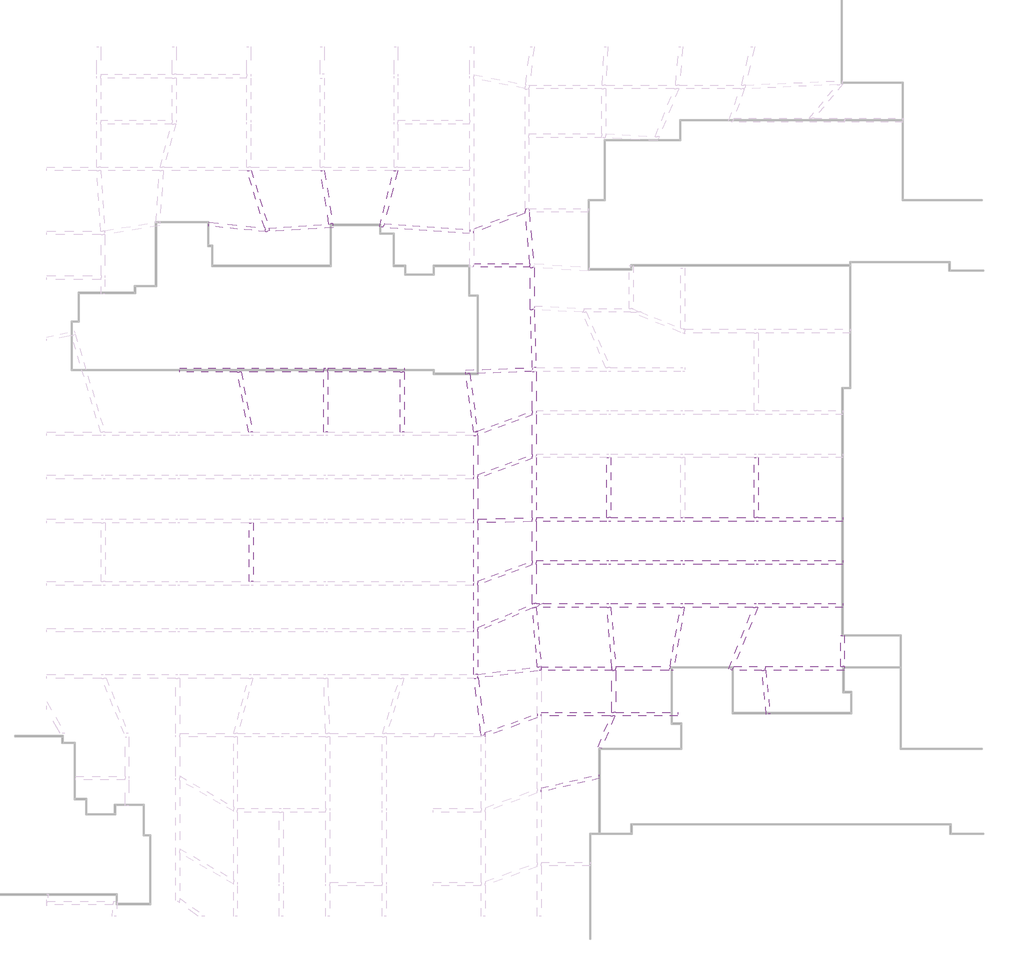
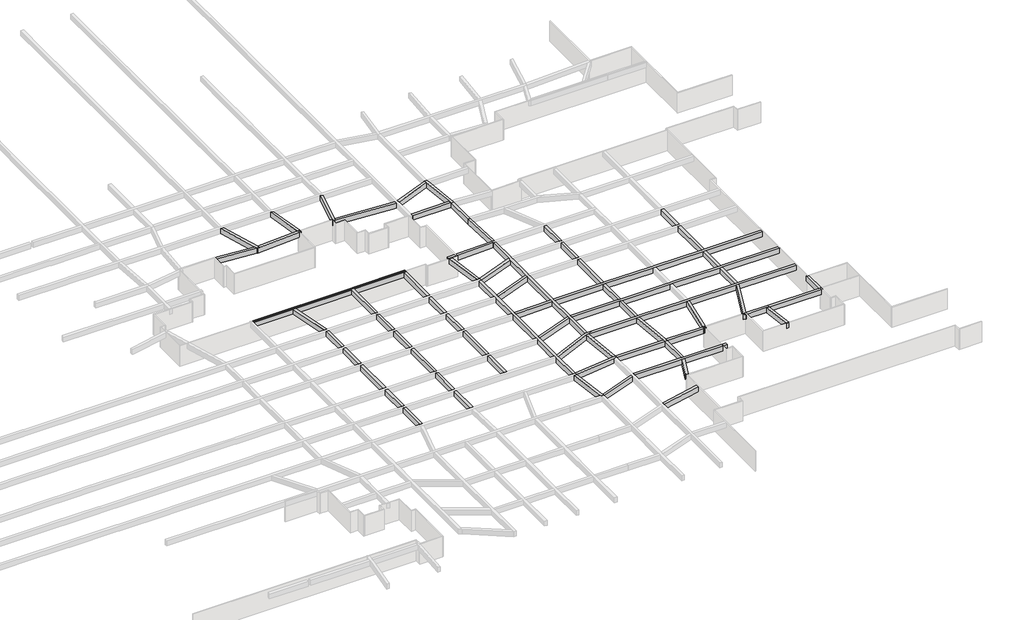
# One storey, part 23 of 45: 48 beams.
"""IFC4 building model written with IfcOpenShell, lengths in millimetres."""

from ifc_helpers import new_model, si_unit, frame, origin, place, context, project, spatial, polyline, outline, extrude, faceted_brep, element, save

model = new_model("IFC4")

# Units and contexts
model_context = context("Model", 3, world=origin())
ifc_project = project(units=[si_unit("LENGTHUNIT", "METRE", prefix="MILLI")], contexts=[model_context])

# Site, building, storey
site = spatial("IfcSite", under=ifc_project)
building = spatial("IfcBuilding", under=site)
storey = spatial("IfcBuildingStorey", under=building, Name="户型图", Elevation=0.0)

# Beams
placement = place(None, origin())
element("IfcBeam", 1, ObjectType="混凝土 - 矩形梁 : KL_beam", at=placement, inside=storey, context=model_context, shape_type="Brep", body=[
    faceted_brep([(31153.9230726, -39503.2652038, 3300.0), (30648.1791725, -33722.5859731, 3300.0), (30613.5574676, -33326.8580756, 3300.0), (30213.5574676, -33344.3224528, 3300.0), (30217.5432201, -33389.8798118, 3300.0), (30253.8104481, -33804.4161248, 3300.0), (30715.2619075, -39078.8304418, 3300.0), (30750.2573729, -39478.8304418, 3300.0), (30753.9230726, -39520.7295809, 3300.0), (30213.5574676, -33344.3224528, 2500.0), (30217.5432201, -33389.8798118, 2500.0), (30253.8104481, -33804.4161248, 2500.0), (30715.2619075, -39078.8304418, 2500.0), (30750.2573729, -39478.8304418, 2500.0), (30753.9230726, -39520.7295809, 2500.0), (30613.5574676, -33326.8580756, 2500.0), (30648.1791725, -33722.5859731, 2500.0), (31153.9230726, -39503.2652038, 2500.0)], [[[0, 1, 2, 3, 4, 5, 6, 7, 8]], [[8, 7, 6, 5, 4, 3, 9, 10, 11, 12, 13, 14]], [[14, 13, 12, 11, 10, 9, 15, 16, 17]], [[2, 1, 0, 17, 16, 15]], [[2, 15, 9, 3]], [[0, 8, 14, 17]]]),
])
element("IfcBeam", 2, ObjectType="混凝土 - 矩形梁 : KL_beam", at=placement, inside=storey, context=model_context, shape_type="Brep", body=[
    faceted_brep([(31153.9230726, -39503.2652038, 3300.0), (30753.9230726, -39520.7295809, 3300.0), (30753.9230726, -43901.7903057, 3300.0), (30760.4408066, -43902.1318857, 3300.0), (31153.9230726, -43922.7534174, 3300.0), (31153.9230726, -43522.204479, 3300.0), (30753.9230726, -39520.7295809, 2500.0), (30753.9230726, -43901.7903057, 2500.0), (31153.9230726, -39503.2652038, 2500.0), (31153.9230726, -43522.204479, 2500.0), (31153.9230726, -43922.7534174, 2500.0), (30760.4408066, -43902.1318857, 2500.0)], [[[0, 1, 2, 3, 4, 5]], [[1, 6, 7, 2]], [[6, 8, 9, 10, 11, 7]], [[8, 0, 5, 4, 10, 9]], [[0, 8, 6, 1]], [[4, 3, 2, 7, 11, 10]]]),
])
element("IfcBeam", 3, ObjectType="混凝土 - 矩形梁 : KL_beam", at=placement, inside=storey, context=model_context, shape_type="SweptSolid", body=[
    extrude(outline(polyline([(1338.0119922, -57112.697306), (1738.0119922, -57112.697306), (1738.0119922, -61244.2645659), (1338.0119922, -61244.2645659), (1338.0119922, -57112.697306)])), frame((0.0, 0.0, 2500.0), z_axis=(0.0, 0.0, 1.0), x_axis=(1.0, 0.0, 0.0)), (0.0, 0.0, 1.0), 800.0),
    extrude(outline(polyline([(1738.0119922, -82134.4617231), (1338.0119922, -82134.4617231), (1338.0119922, -77689.9052253), (1738.0119922, -77689.9052253), (1738.0119922, -82134.4617231)])), frame((0.0, 0.0, 2500.0), z_axis=(0.0, 0.0, 1.0), x_axis=(1.0, 0.0, 0.0)), (0.0, 0.0, 1.0), 800.0),
    extrude(outline(polyline([(1338.0119922, -61644.2645659), (1738.0119922, -61644.2645659), (1738.0119922, -65862.2662437), (1338.0119922, -65862.2662437), (1338.0119922, -61644.2645659)])), frame((0.0, 0.0, 2500.0), z_axis=(0.0, 0.0, 1.0), x_axis=(1.0, 0.0, 0.0)), (0.0, 0.0, 1.0), 800.0),
    extrude(outline(polyline([(1338.0119922, -66262.2662437), (1738.0119922, -66262.2662437), (1738.0119922, -72411.6769994), (1338.0119922, -72411.6769994), (1338.0119922, -66262.2662437)])), frame((0.0, 0.0, 2500.0), z_axis=(0.0, 0.0, 1.0), x_axis=(1.0, 0.0, 0.0)), (0.0, 0.0, 1.0), 800.0),
    extrude(outline(polyline([(1338.0119922, -72811.6769994), (1738.0119922, -72811.6769994), (1738.0119922, -77289.9052253), (1338.0119922, -77289.9052253), (1338.0119922, -72811.6769994)])), frame((0.0, 0.0, 2500.0), z_axis=(0.0, 0.0, 1.0), x_axis=(1.0, 0.0, 0.0)), (0.0, 0.0, 1.0), 800.0),
])
element("IfcBeam", 4, ObjectType="混凝土 - 矩形梁 : KL_beam", at=placement, inside=storey, context=model_context, shape_type="Brep", body=[
    faceted_brep([(9138.0119922, -82134.4617231, 3300.0), (9538.0119922, -82134.4617231, 3300.0), (9538.0119922, -77689.9052253, 3300.0), (9138.0119922, -77689.9052253, 3300.0), (9538.0119922, -82134.4617231, 2500.0), (9538.0119922, -77689.9052253, 2500.0), (9138.0119922, -82134.4617231, 2500.0), (9138.0119922, -77689.9052253, 2500.0)], [[[0, 1, 2, 3]], [[1, 4, 5, 2]], [[4, 6, 7, 5]], [[6, 0, 3, 7]], [[1, 0, 6, 4]], [[3, 2, 5, 7]]]),
    faceted_brep([(9138.0119922, -57112.697306, 3300.0), (9538.0119922, -57112.697306, 3300.0), (9538.0119922, -57112.697306, 2500.0), (9138.0119922, -57112.697306, 2500.0), (9538.0119922, -61244.2645659, 3300.0), (9138.0119922, -61244.2645659, 3300.0), (9138.0119922, -61244.2645659, 2500.0), (9538.0119922, -61244.2645659, 2500.0)], [[[0, 1, 2, 3]], [[4, 5, 6, 7]], [[1, 0, 5, 4]], [[2, 1, 4, 7]], [[3, 2, 7, 6]], [[0, 3, 6, 5]]]),
    faceted_brep([(9538.0119922, -56712.697306, 3300.0), (9138.0119922, -56712.697306, 3300.0), (9138.0119922, -56712.697306, 2500.0), (9538.0119922, -56712.697306, 2500.0), (9538.0119922, -50434.4617231, 3300.0), (9538.0119922, -50034.4617231, 3300.0), (9138.0119922, -50034.4617231, 3300.0), (9138.0119922, -50434.4617231, 3300.0), (9538.0119922, -50434.4617231, 2500.0), (9538.0119922, -50034.4617231, 2500.0), (9138.0119922, -50434.4617231, 2500.0), (9138.0119922, -50034.4617231, 2500.0)], [[[0, 1, 2, 3]], [[1, 0, 4, 5, 6, 7]], [[0, 3, 8, 9, 5, 4]], [[3, 2, 10, 11, 9, 8]], [[2, 1, 7, 6, 11, 10]], [[6, 5, 9, 11]]]),
    faceted_brep([(9138.0119922, -61644.2645659, 3300.0), (9538.0119922, -61644.2645659, 3300.0), (9538.0119922, -61644.2645659, 2500.0), (9138.0119922, -61644.2645659, 2500.0), (9538.0119922, -65862.2662437, 3300.0), (9138.0119922, -65862.2662437, 3300.0), (9138.0119922, -65862.2662437, 2500.0), (9538.0119922, -65862.2662437, 2500.0)], [[[0, 1, 2, 3]], [[4, 5, 6, 7]], [[1, 0, 5, 4]], [[2, 1, 4, 7]], [[3, 2, 7, 6]], [[0, 3, 6, 5]]]),
    faceted_brep([(9138.0119922, -66262.2662437, 3300.0), (9538.0119922, -66262.2662437, 3300.0), (9538.0119922, -66262.2662437, 2500.0), (9138.0119922, -66262.2662437, 2500.0), (9538.0119922, -72411.6769994, 3300.0), (9138.0119922, -72411.6769994, 3300.0), (9138.0119922, -72411.6769994, 2500.0), (9538.0119922, -72411.6769994, 2500.0)], [[[0, 1, 2, 3]], [[4, 5, 6, 7]], [[1, 0, 5, 4]], [[2, 1, 4, 7]], [[3, 2, 7, 6]], [[0, 3, 6, 5]]]),
    faceted_brep([(9138.0119922, -72811.6769994, 3300.0), (9538.0119922, -72811.6769994, 3300.0), (9538.0119922, -72811.6769994, 2500.0), (9138.0119922, -72811.6769994, 2500.0), (9538.0119922, -77289.9052253, 3300.0), (9138.0119922, -77289.9052253, 3300.0), (9138.0119922, -77289.9052253, 2500.0), (9538.0119922, -77289.9052253, 2500.0)], [[[0, 1, 2, 3]], [[4, 5, 6, 7]], [[1, 0, 5, 4]], [[2, 1, 4, 7]], [[3, 2, 7, 6]], [[0, 3, 6, 5]]]),
])
element("IfcBeam", 5, ObjectType="混凝土 - 矩形梁 : KL_beam", at=placement, inside=storey, context=model_context, shape_type="Brep", body=[
    faceted_brep([(17560.5867178, -50434.4617231, 3300.0), (17560.5867178, -50034.4617231, 3300.0), (9538.0119922, -50034.4617231, 3300.0), (9538.0119922, -50434.4617231, 3300.0), (17160.5867178, -50434.4617231, 3300.0), (17560.5867178, -50434.4617231, 2500.0), (9538.0119922, -50434.4617231, 2500.0), (17160.5867178, -50434.4617231, 2500.0), (17560.5867178, -50034.4617231, 2500.0), (9538.0119922, -50034.4617231, 2500.0)], [[[0, 1, 2, 3, 4]], [[5, 0, 4, 3, 6, 7]], [[8, 5, 7, 6, 9]], [[1, 8, 9, 2]], [[3, 2, 9, 6]], [[1, 0, 5, 8]]]),
])
element("IfcBeam", 6, ObjectType="混凝土 - 矩形梁 : KL_beam", at=placement, inside=storey, context=model_context, shape_type="Brep", body=[
    faceted_brep([(-5961.9880078, -50034.4617231, 3300.0), (-5961.9880078, -50434.4617231, 3300.0), (74.9529241, -50434.4617231, 3300.0), (482.4396021, -50434.4617231, 3300.0), (9138.0119922, -50434.4617231, 3300.0), (9138.0119922, -50034.4617231, 3300.0), (-5961.9880078, -50034.4617231, 2500.0), (9138.0119922, -50034.4617231, 2500.0), (-5961.9880078, -50434.4617231, 2500.0), (9138.0119922, -50434.4617231, 2500.0), (482.4396021, -50434.4617231, 2500.0), (74.9529241, -50434.4617231, 2500.0)], [[[0, 1, 2, 3, 4, 5]], [[6, 0, 5, 7]], [[8, 6, 7, 9, 10, 11]], [[1, 8, 11, 10, 9, 4, 3, 2]], [[1, 0, 6, 8]], [[5, 4, 9, 7]]]),
])
element("IfcBeam", 7, ObjectType="混凝土 - 矩形梁 : KL_beam", at=placement, inside=storey, context=model_context, shape_type="SweptSolid", body=[
    extrude(outline(polyline([(1702.8049756, -56712.697306), (1295.3182976, -56712.697306), (74.9529241, -50434.4617231), (482.4396021, -50434.4617231), (1702.8049756, -56712.697306)])), frame((0.0, 0.0, 2500.0), z_axis=(0.0, 0.0, 1.0), x_axis=(1.0, 0.0, 0.0)), (0.0, 0.0, 1.0), 800.0),
])
element("IfcBeam", 8, ObjectType="混凝土 - 矩形梁 : KL_beam", at=placement, inside=storey, context=model_context, shape_type="SweptSolid", body=[
    extrude(outline(polyline([(17560.5867178, -77289.9052253), (17160.5867178, -77289.9052253), (17160.5867178, -72811.6769994), (17560.5867178, -72811.6769994), (17560.5867178, -77289.9052253)])), frame((0.0, 0.0, 2500.0), z_axis=(0.0, 0.0, 1.0), x_axis=(1.0, 0.0, 0.0)), (0.0, 0.0, 1.0), 800.0),
    extrude(outline(polyline([(17160.5867178, -50434.4617231), (17560.5867178, -50434.4617231), (17560.5867178, -56712.697306), (17160.5867178, -56712.697306), (17160.5867178, -50434.4617231)])), frame((0.0, 0.0, 2500.0), z_axis=(0.0, 0.0, 1.0), x_axis=(1.0, 0.0, 0.0)), (0.0, 0.0, 1.0), 800.0),
    extrude(outline(polyline([(17160.5867178, -57112.697306), (17560.5867178, -57112.697306), (17560.5867178, -61244.2645659), (17160.5867178, -61244.2645659), (17160.5867178, -57112.697306)])), frame((0.0, 0.0, 2500.0), z_axis=(0.0, 0.0, 1.0), x_axis=(1.0, 0.0, 0.0)), (0.0, 0.0, 1.0), 800.0),
    extrude(outline(polyline([(17160.5867178, -61644.2645659), (17560.5867178, -61644.2645659), (17560.5867178, -65862.2662437), (17160.5867178, -65862.2662437), (17160.5867178, -61644.2645659)])), frame((0.0, 0.0, 2500.0), z_axis=(0.0, 0.0, 1.0), x_axis=(1.0, 0.0, 0.0)), (0.0, 0.0, 1.0), 800.0),
    extrude(outline(polyline([(17160.5867178, -66262.2662437), (17560.5867178, -66262.2662437), (17560.5867178, -72411.6769994), (17160.5867178, -72411.6769994), (17160.5867178, -66262.2662437)])), frame((0.0, 0.0, 2500.0), z_axis=(0.0, 0.0, 1.0), x_axis=(1.0, 0.0, 0.0)), (0.0, 0.0, 1.0), 800.0),
])
element("IfcBeam", 9, ObjectType="混凝土 - 矩形梁 : KL_beam", at=placement, inside=storey, context=model_context, shape_type="Brep", body=[
    faceted_brep([(25266.4388689, -57112.697306, 3300.0), (24866.4388689, -57112.697306, 3300.0), (24866.4388689, -61244.2645659, 3300.0), (24866.4388689, -61644.2645659, 3300.0), (24866.4388689, -65862.2662437, 3300.0), (24866.4388689, -66262.2662437, 3300.0), (24866.4388689, -72411.6769994, 3300.0), (24866.4388689, -72811.6769994, 3300.0), (24866.4388689, -77289.9052253, 3300.0), (24866.4388689, -77689.9052253, 3300.0), (24866.4388689, -82134.4617231, 3300.0), (25266.4388689, -82134.4617231, 3300.0), (25266.4388689, -82108.4028459, 3300.0), (25266.4388689, -77622.2823376, 3300.0), (25266.4388689, -77187.7381866, 3300.0), (25266.4388689, -72751.6932425, 3300.0), (25266.4388689, -72326.0221335, 3300.0), (25266.4388689, -66257.3977389, 3300.0), (25266.4388689, -65857.2762703, 3300.0), (25266.4388689, -61584.3060735, 3300.0), (25266.4388689, -61158.6349646, 3300.0), (25266.4388689, -57112.697306, 2500.0), (25266.4388689, -82134.4617231, 2500.0), (25266.4388689, -82108.4028459, 2500.0), (25266.4388689, -77622.2823376, 2500.0), (25266.4388689, -77187.7381866, 2500.0), (25266.4388689, -72751.6932425, 2500.0), (25266.4388689, -72326.0221335, 2500.0), (25266.4388689, -66257.3977389, 2500.0), (25266.4388689, -65857.2762703, 2500.0), (25266.4388689, -61584.3060735, 2500.0), (25266.4388689, -61158.6349646, 2500.0), (24866.4388689, -57112.697306, 2500.0), (24866.4388689, -82134.4617231, 2500.0), (24866.4388689, -77689.9052253, 2500.0), (24866.4388689, -77289.9052253, 2500.0), (24866.4388689, -72811.6769994, 2500.0), (24866.4388689, -72411.6769994, 2500.0), (24866.4388689, -66262.2662437, 2500.0), (24866.4388689, -65862.2662437, 2500.0), (24866.4388689, -61644.2645659, 2500.0), (24866.4388689, -61244.2645659, 2500.0)], [[[0, 1, 2, 3, 4, 5, 6, 7, 8, 9, 10, 11, 12, 13, 14, 15, 16, 17, 18, 19, 20]], [[21, 0, 20, 19, 18, 17, 16, 15, 14, 13, 12, 11, 22, 23, 24, 25, 26, 27, 28, 29, 30, 31]], [[32, 21, 31, 30, 29, 28, 27, 26, 25, 24, 23, 22, 33, 34, 35, 36, 37, 38, 39, 40, 41]], [[1, 32, 41, 40, 39, 38, 37, 36, 35, 34, 33, 10, 9, 8, 7, 6, 5, 4, 3, 2]], [[1, 0, 21, 32]], [[11, 10, 33, 22]]]),
])
element("IfcBeam", 10, ObjectType="混凝土 - 矩形梁 : KL_beam", at=placement, inside=storey, context=model_context, shape_type="Brep", body=[
    faceted_brep([(25031.1734727, -56712.697306, 3300.0), (25266.4388689, -56712.697306, 3300.0), (25266.4388689, -57052.7388136, 3300.0), (30980.1331881, -54973.1241538, 3300.0), (30980.1331881, -54547.4530448, 3300.0), (25230.8624807, -56640.016451, 3300.0), (25266.4388689, -57052.7388136, 2500.0), (30980.1331881, -54973.1241538, 2500.0), (25266.4388689, -56712.697306, 2500.0), (25031.1734727, -56712.697306, 2500.0), (25230.8624807, -56640.016451, 2500.0), (30980.1331881, -54547.4530448, 2500.0)], [[[0, 1, 2, 3, 4, 5]], [[2, 6, 7, 3]], [[8, 9, 10, 11, 7, 6]], [[9, 0, 5, 4, 11, 10]], [[8, 1, 0, 9]], [[1, 8, 6, 2]], [[4, 3, 7, 11]]]),
])
element("IfcBeam", 11, ObjectType="混凝土 - 矩形梁 : KL_beam", at=placement, inside=storey, context=model_context, shape_type="SweptSolid", body=[
    extrude(outline(polyline([(25266.4388689, -61584.3060735), (25266.4388689, -61158.6349646), (30980.1331881, -59079.0203047), (30980.1331881, -59504.6914136), (25266.4388689, -61584.3060735)])), frame((0.0, 0.0, 2500.0), z_axis=(0.0, 0.0, 1.0), x_axis=(1.0, 0.0, 0.0)), (0.0, 0.0, 1.0), 800.0),
])
element("IfcBeam", 12, ObjectType="混凝土 - 矩形梁 : KL_beam", at=placement, inside=storey, context=model_context, shape_type="SweptSolid", body=[
    extrude(outline(polyline([(25266.4388689, -66257.3977389), (25266.4388689, -65857.2762703), (30980.1331881, -65716.4554426), (30980.1331881, -66116.5769112), (25266.4388689, -66257.3977389)])), frame((0.0, 0.0, 2500.0), z_axis=(0.0, 0.0, 1.0), x_axis=(1.0, 0.0, 0.0)), (0.0, 0.0, 1.0), 800.0),
])
element("IfcBeam", 13, ObjectType="混凝土 - 矩形梁 : KL_beam", at=placement, inside=storey, context=model_context, shape_type="SweptSolid", body=[
    extrude(outline(polyline([(25266.4388689, -72751.6932425), (25266.4388689, -72326.0221335), (30980.1331881, -70246.4074737), (30980.1331881, -70672.0785826), (25266.4388689, -72751.6932425)])), frame((0.0, 0.0, 2500.0), z_axis=(0.0, 0.0, 1.0), x_axis=(1.0, 0.0, 0.0)), (0.0, 0.0, 1.0), 800.0),
])
element("IfcBeam", 14, ObjectType="混凝土 - 矩形梁 : KL_beam", at=placement, inside=storey, context=model_context, shape_type="Brep", body=[
    faceted_brep([(32124.8023079, -74711.0797773, 3300.0), (31380.1331881, -74711.0797773, 3300.0), (31101.0804418, -74711.0797773, 3300.0), (30980.1331881, -74762.4188406, 3300.0), (25266.4388689, -77187.7381866, 3300.0), (25266.4388689, -77622.2823376, 3300.0), (31001.9328556, -75187.7095817, 3300.0), (31182.4613615, -75111.0797773, 3300.0), (32124.8023079, -74711.0797773, 2500.0), (25266.4388689, -77622.2823376, 2500.0), (31001.9328556, -75187.7095817, 2500.0), (31182.4613615, -75111.0797773, 2500.0), (31101.0804418, -74711.0797773, 2500.0), (31380.1331881, -74711.0797773, 2500.0), (25266.4388689, -77187.7381866, 2500.0), (30980.1331881, -74762.4188406, 2500.0)], [[[0, 1, 2, 3, 4, 5, 6, 7]], [[8, 0, 7, 6, 5, 9, 10, 11]], [[12, 13, 8, 11, 10, 9, 14, 15]], [[2, 12, 15, 14, 4, 3]], [[5, 4, 14, 9]], [[2, 1, 0, 8, 13, 12]]]),
])
element("IfcBeam", 15, ObjectType="混凝土 - 矩形梁 : KL_beam", at=placement, inside=storey, context=model_context, shape_type="Brep", body=[
    faceted_brep([(25266.4388689, -82108.4028459, 3300.0), (25266.4388689, -82134.4617231, 3300.0), (25266.4388689, -82511.406776, 3300.0), (25289.3682002, -82508.5914082, 3300.0), (31516.4740744, -81743.9989477, 3300.0), (31916.4740744, -81694.8851233, 3300.0), (31931.3727413, -81693.0557971, 3300.0), (31916.4740744, -81509.5363909, 3300.0), (31900.9194594, -81317.9371223, 3300.0), (31898.9785552, -81294.0293728, 3300.0), (31501.6234284, -81342.8184476, 3300.0), (25266.4388689, -82511.406776, 2500.0), (25289.3682002, -82508.5914082, 2500.0), (31516.4740744, -81743.9989477, 2500.0), (31916.4740744, -81694.8851233, 2500.0), (31931.3727413, -81693.0557971, 2500.0), (25266.4388689, -82134.4617231, 2500.0), (25266.4388689, -82108.4028459, 2500.0), (31501.6234284, -81342.8184476, 2500.0), (31898.9785552, -81294.0293728, 2500.0), (31900.9194594, -81317.9371223, 2500.0), (31916.4740744, -81509.5363909, 2500.0)], [[[0, 1, 2, 3, 4, 5, 6, 7, 8, 9, 10]], [[2, 11, 12, 13, 14, 15, 6, 5, 4, 3]], [[11, 16, 17, 18, 19, 20, 21, 15, 14, 13, 12]], [[9, 19, 18, 17, 0, 10]], [[0, 17, 16, 11, 2, 1]], [[9, 8, 7, 6, 15, 21, 20, 19]]]),
])
element("IfcBeam", 16, ObjectType="混凝土 - 矩形梁 : KL_beam", at=placement, inside=storey, context=model_context, shape_type="Brep", body=[
    faceted_brep([(63459.1246226, -74711.0797773, 3300.0), (63459.1246226, -75111.0797773, 3300.0), (63459.1246226, -75111.0797773, 2500.0), (63459.1246226, -74711.0797773, 2500.0), (54624.1889168, -74711.0797773, 3300.0), (54224.1889168, -74711.0797773, 3300.0), (46924.1889168, -74711.0797773, 3300.0), (46524.1889168, -74711.0797773, 3300.0), (39180.1331881, -74711.0797773, 3300.0), (38780.1331881, -74711.0797773, 3300.0), (32124.8023079, -74711.0797773, 3300.0), (31182.4613615, -75111.0797773, 3300.0), (31397.0277867, -75111.0797773, 3300.0), (38795.7118136, -75111.0797773, 3300.0), (39197.0277867, -75111.0797773, 3300.0), (46485.8381983, -75111.0797773, 3300.0), (46892.008843, -75111.0797773, 3300.0), (54127.6767231, -75111.0797773, 3300.0), (54559.0906202, -75111.0797773, 3300.0), (31182.4613615, -75111.0797773, 2500.0), (31397.0277867, -75111.0797773, 2500.0), (38795.7118136, -75111.0797773, 2500.0), (39197.0277867, -75111.0797773, 2500.0), (46485.8381983, -75111.0797773, 2500.0), (46892.008843, -75111.0797773, 2500.0), (54127.6767231, -75111.0797773, 2500.0), (54559.0906202, -75111.0797773, 2500.0), (32124.8023079, -74711.0797773, 2500.0), (38780.1331881, -74711.0797773, 2500.0), (39180.1331881, -74711.0797773, 2500.0), (46524.1889168, -74711.0797773, 2500.0), (46924.1889168, -74711.0797773, 2500.0), (54224.1889168, -74711.0797773, 2500.0), (54624.1889168, -74711.0797773, 2500.0)], [[[0, 1, 2, 3]], [[1, 0, 4, 5, 6, 7, 8, 9, 10, 11, 12, 13, 14, 15, 16, 17, 18]], [[2, 1, 18, 17, 16, 15, 14, 13, 12, 11, 19, 20, 21, 22, 23, 24, 25, 26]], [[3, 2, 26, 25, 24, 23, 22, 21, 20, 19, 27, 28, 29, 30, 31, 32, 33]], [[0, 3, 33, 32, 31, 30, 29, 28, 27, 10, 9, 8, 7, 6, 5, 4]], [[11, 10, 27, 19]]]),
])
element("IfcBeam", 17, ObjectType="混凝土 - 矩形梁 : KL_beam", at=placement, inside=storey, context=model_context, shape_type="Brep", body=[
    faceted_brep([(63459.3057658, -70188.5460678, 3300.0), (63459.3057658, -70588.5460678, 3300.0), (63459.3057658, -70588.5460678, 2500.0), (63459.3057658, -70188.5460678, 2500.0), (54624.1889168, -70188.5460678, 3300.0), (54224.1889168, -70188.5460678, 3300.0), (46924.1889168, -70188.5460678, 3300.0), (46524.1889168, -70188.5460678, 3300.0), (39180.1331881, -70188.5460678, 3300.0), (38780.1331881, -70188.5460678, 3300.0), (31380.1331881, -70188.5460678, 3300.0), (31380.1331881, -70588.5460678, 3300.0), (38780.1331881, -70588.5460678, 3300.0), (39180.1331881, -70588.5460678, 3300.0), (46524.1889168, -70588.5460678, 3300.0), (46924.1889168, -70588.5460678, 3300.0), (54224.1889168, -70588.5460678, 3300.0), (54624.1889168, -70588.5460678, 3300.0), (31380.1331881, -70588.5460678, 2500.0), (38780.1331881, -70588.5460678, 2500.0), (39180.1331881, -70588.5460678, 2500.0), (46524.1889168, -70588.5460678, 2500.0), (46924.1889168, -70588.5460678, 2500.0), (54224.1889168, -70588.5460678, 2500.0), (54624.1889168, -70588.5460678, 2500.0), (31380.1331881, -70188.5460678, 2500.0), (38780.1331881, -70188.5460678, 2500.0), (39180.1331881, -70188.5460678, 2500.0), (46524.1889168, -70188.5460678, 2500.0), (46924.1889168, -70188.5460678, 2500.0), (54224.1889168, -70188.5460678, 2500.0), (54624.1889168, -70188.5460678, 2500.0)], [[[0, 1, 2, 3]], [[1, 0, 4, 5, 6, 7, 8, 9, 10, 11, 12, 13, 14, 15, 16, 17]], [[2, 1, 17, 16, 15, 14, 13, 12, 11, 18, 19, 20, 21, 22, 23, 24]], [[3, 2, 24, 23, 22, 21, 20, 19, 18, 25, 26, 27, 28, 29, 30, 31]], [[0, 3, 31, 30, 29, 28, 27, 26, 25, 10, 9, 8, 7, 6, 5, 4]], [[10, 25, 18, 11]]]),
])
element("IfcBeam", 18, ObjectType="混凝土 - 矩形梁 : KL_beam", at=placement, inside=storey, context=model_context, shape_type="Brep", body=[
    faceted_brep([(63459.3057658, -65711.9700913, 3300.0), (63459.3057658, -66111.9700913, 3300.0), (63459.3057658, -66111.9700913, 2500.0), (63459.3057658, -65711.9700913, 2500.0), (54624.1889168, -65711.9700913, 3300.0), (54224.1889168, -65711.9700913, 3300.0), (46924.1889168, -65711.9700913, 3300.0), (46524.1889168, -65711.9700913, 3300.0), (39180.1331881, -65711.9700913, 3300.0), (38780.1331881, -65711.9700913, 3300.0), (31380.1331881, -65711.9700913, 3300.0), (31380.1331881, -66111.9700913, 3300.0), (38780.1331881, -66111.9700913, 3300.0), (39180.1331881, -66111.9700913, 3300.0), (46524.1889168, -66111.9700913, 3300.0), (46924.1889168, -66111.9700913, 3300.0), (54224.1889168, -66111.9700913, 3300.0), (54624.1889168, -66111.9700913, 3300.0), (31380.1331881, -66111.9700913, 2500.0), (38780.1331881, -66111.9700913, 2500.0), (39180.1331881, -66111.9700913, 2500.0), (46524.1889168, -66111.9700913, 2500.0), (46924.1889168, -66111.9700913, 2500.0), (54224.1889168, -66111.9700913, 2500.0), (54624.1889168, -66111.9700913, 2500.0), (31380.1331881, -65711.9700913, 2500.0), (38780.1331881, -65711.9700913, 2500.0), (39180.1331881, -65711.9700913, 2500.0), (46524.1889168, -65711.9700913, 2500.0), (46924.1889168, -65711.9700913, 2500.0), (54224.1889168, -65711.9700913, 2500.0), (54624.1889168, -65711.9700913, 2500.0)], [[[0, 1, 2, 3]], [[1, 0, 4, 5, 6, 7, 8, 9, 10, 11, 12, 13, 14, 15, 16, 17]], [[2, 1, 17, 16, 15, 14, 13, 12, 11, 18, 19, 20, 21, 22, 23, 24]], [[3, 2, 24, 23, 22, 21, 20, 19, 18, 25, 26, 27, 28, 29, 30, 31]], [[0, 3, 31, 30, 29, 28, 27, 26, 25, 10, 9, 8, 7, 6, 5, 4]], [[10, 25, 18, 11]]]),
])
element("IfcBeam", 19, ObjectType="混凝土 - 矩形梁 : KL_beam", at=placement, inside=storey, context=model_context, shape_type="Brep", body=[
    faceted_brep([(31161.4184615, -43923.1462341, 3300.0), (31153.9230726, -43922.7534174, 3300.0), (30760.4408066, -43902.1318857, 3300.0), (30973.0187032, -49989.5663744, 3300.0), (31373.2625209, -49989.5663744, 3300.0), (30760.4408066, -43902.1318857, 2500.0), (30973.0187032, -49989.5663744, 2500.0), (31153.9230726, -43922.7534174, 2500.0), (31161.4184615, -43923.1462341, 2500.0), (31373.2625209, -49989.5663744, 2500.0)], [[[0, 1, 2, 3, 4]], [[2, 5, 6, 3]], [[5, 7, 8, 9, 6]], [[8, 0, 4, 9]], [[5, 2, 1, 0, 8, 7]], [[4, 3, 6, 9]]]),
])
element("IfcBeam", 20, ObjectType="混凝土 - 矩形梁 : KL_beam", at=placement, inside=storey, context=model_context, shape_type="Brep", body=[
    faceted_brep([(31380.1331881, -50389.5663744, 3300.0), (30980.1331881, -50389.5663744, 3300.0), (30980.1331881, -50396.672143, 3300.0), (30980.1331881, -54547.4530448, 3300.0), (30980.1331881, -54973.1241538, 3300.0), (30980.1331881, -59079.0203047, 3300.0), (30980.1331881, -59504.6914136, 3300.0), (30980.1331881, -65716.4554426, 3300.0), (30980.1331881, -66116.5769112, 3300.0), (30980.1331881, -70246.4074737, 3300.0), (30980.1331881, -70672.0785826, 3300.0), (30980.1331881, -74762.4188406, 3300.0), (31101.0804418, -74711.0797773, 3300.0), (31380.1331881, -74711.0797773, 3300.0), (31380.1331881, -70588.5460678, 3300.0), (31380.1331881, -70188.5460678, 3300.0), (31380.1331881, -66111.9700913, 3300.0), (31380.1331881, -65711.9700913, 3300.0), (31380.1331881, -59421.1336343, 3300.0), (31380.1331881, -59021.1336343, 3300.0), (31380.1331881, -54889.5663744, 3300.0), (31380.1331881, -54489.5663744, 3300.0), (30980.1331881, -50389.5663744, 2500.0), (30980.1331881, -50396.672143, 2500.0), (30980.1331881, -54547.4530448, 2500.0), (30980.1331881, -54973.1241538, 2500.0), (30980.1331881, -59079.0203047, 2500.0), (30980.1331881, -59504.6914136, 2500.0), (30980.1331881, -65716.4554426, 2500.0), (30980.1331881, -66116.5769112, 2500.0), (30980.1331881, -70246.4074737, 2500.0), (30980.1331881, -70672.0785826, 2500.0), (30980.1331881, -74762.4188406, 2500.0), (31380.1331881, -50389.5663744, 2500.0), (31380.1331881, -54489.5663744, 2500.0), (31380.1331881, -54889.5663744, 2500.0), (31380.1331881, -59021.1336343, 2500.0), (31380.1331881, -59421.1336343, 2500.0), (31380.1331881, -65711.9700913, 2500.0), (31380.1331881, -66111.9700913, 2500.0), (31380.1331881, -70188.5460678, 2500.0), (31380.1331881, -70588.5460678, 2500.0), (31380.1331881, -74711.0797773, 2500.0), (31101.0804418, -74711.0797773, 2500.0)], [[[0, 1, 2, 3, 4, 5, 6, 7, 8, 9, 10, 11, 12, 13, 14, 15, 16, 17, 18, 19, 20, 21]], [[1, 22, 23, 24, 25, 26, 27, 28, 29, 30, 31, 32, 11, 10, 9, 8, 7, 6, 5, 4, 3, 2]], [[22, 33, 34, 35, 36, 37, 38, 39, 40, 41, 42, 43, 32, 31, 30, 29, 28, 27, 26, 25, 24, 23]], [[33, 0, 21, 20, 19, 18, 17, 16, 15, 14, 13, 42, 41, 40, 39, 38, 37, 36, 35, 34]], [[1, 0, 33, 22]], [[12, 43, 42, 13]], [[43, 12, 11, 32]]]),
])
element("IfcBeam", 21, ObjectType="混凝土 - 矩形梁 : KL_beam", at=placement, inside=storey, context=model_context, shape_type="Brep", body=[
    faceted_brep([(31501.6234284, -81342.8184476, 3300.0), (31898.9785552, -81294.0293728, 3300.0), (31397.0277867, -75111.0797773, 3300.0), (31380.1331881, -75111.0797773, 3300.0), (31182.4613615, -75111.0797773, 3300.0), (31001.9328556, -75187.7095817, 3300.0), (31501.6234284, -81342.8184476, 2500.0), (31001.9328556, -75187.7095817, 2500.0), (31898.9785552, -81294.0293728, 2500.0), (31182.4613615, -75111.0797773, 2500.0), (31380.1331881, -75111.0797773, 2500.0), (31397.0277867, -75111.0797773, 2500.0)], [[[0, 1, 2, 3, 4, 5]], [[6, 0, 5, 7]], [[8, 6, 7, 9, 10, 11]], [[1, 8, 11, 2]], [[1, 0, 6, 8]], [[2, 11, 10, 9, 4, 3]], [[5, 4, 9, 7]]]),
])
element("IfcBeam", 22, ObjectType="混凝土 - 矩形梁 : KL_beam", at=placement, inside=storey, context=model_context, shape_type="SweptSolid", body=[
    extrude(outline(polyline([(39180.1331881, -74711.0797773), (38780.1331881, -74711.0797773), (38780.1331881, -70588.5460678), (39180.1331881, -70588.5460678), (39180.1331881, -74711.0797773)])), frame((0.0, 0.0, 2500.0), z_axis=(0.0, 0.0, 1.0), x_axis=(1.0, 0.0, 0.0)), (0.0, 0.0, 1.0), 800.0),
    extrude(outline(polyline([(38780.1331881, -50389.5663744), (39180.1331881, -50389.5663744), (39180.1331881, -54489.5663744), (38780.1331881, -54489.5663744), (38780.1331881, -50389.5663744)])), frame((0.0, 0.0, 2500.0), z_axis=(0.0, 0.0, 1.0), x_axis=(1.0, 0.0, 0.0)), (0.0, 0.0, 1.0), 800.0),
    extrude(outline(polyline([(39180.1331881, -70188.5460678), (38780.1331881, -70188.5460678), (38780.1331881, -66111.9700913), (39180.1331881, -66111.9700913), (39180.1331881, -70188.5460678)])), frame((0.0, 0.0, 2500.0), z_axis=(0.0, 0.0, 1.0), x_axis=(1.0, 0.0, 0.0)), (0.0, 0.0, 1.0), 800.0),
    extrude(outline(polyline([(39180.1331881, -65711.9700913), (38780.1331881, -65711.9700913), (38780.1331881, -59421.1336343), (39180.1331881, -59421.1336343), (39180.1331881, -65711.9700913)])), frame((0.0, 0.0, 2500.0), z_axis=(0.0, 0.0, 1.0), x_axis=(1.0, 0.0, 0.0)), (0.0, 0.0, 1.0), 800.0),
    extrude(outline(polyline([(39180.1331881, -59021.1336343), (38780.1331881, -59021.1336343), (38780.1331881, -54889.5663744), (39180.1331881, -54889.5663744), (39180.1331881, -59021.1336343)])), frame((0.0, 0.0, 2500.0), z_axis=(0.0, 0.0, 1.0), x_axis=(1.0, 0.0, 0.0)), (0.0, 0.0, 1.0), 800.0),
])
element("IfcBeam", 23, ObjectType="混凝土 - 矩形梁 : KL_beam", at=placement, inside=storey, context=model_context, shape_type="SweptSolid", body=[
    extrude(outline(polyline([(54624.1889168, -74711.0797773), (54224.1889168, -74711.0797773), (54224.1889168, -70588.5460678), (54624.1889168, -70588.5460678), (54624.1889168, -74711.0797773)])), frame((0.0, 0.0, 2500.0), z_axis=(0.0, 0.0, 1.0), x_axis=(1.0, 0.0, 0.0)), (0.0, 0.0, 1.0), 800.0),
    extrude(outline(polyline([(54224.1889168, -54889.5663744), (54624.1889168, -54889.5663744), (54624.1889168, -59021.1336343), (54224.1889168, -59021.1336343), (54224.1889168, -54889.5663744)])), frame((0.0, 0.0, 2500.0), z_axis=(0.0, 0.0, 1.0), x_axis=(1.0, 0.0, 0.0)), (0.0, 0.0, 1.0), 800.0),
    extrude(outline(polyline([(54624.1889168, -70188.5460678), (54224.1889168, -70188.5460678), (54224.1889168, -66111.9700913), (54624.1889168, -66111.9700913), (54624.1889168, -70188.5460678)])), frame((0.0, 0.0, 2500.0), z_axis=(0.0, 0.0, 1.0), x_axis=(1.0, 0.0, 0.0)), (0.0, 0.0, 1.0), 800.0),
    extrude(outline(polyline([(54624.1889168, -65711.9700913), (54224.1889168, -65711.9700913), (54224.1889168, -59421.1336343), (54624.1889168, -59421.1336343), (54624.1889168, -65711.9700913)])), frame((0.0, 0.0, 2500.0), z_axis=(0.0, 0.0, 1.0), x_axis=(1.0, 0.0, 0.0)), (0.0, 0.0, 1.0), 800.0),
])
element("IfcBeam", 24, ObjectType="混凝土 - 矩形梁 : KL_beam", at=placement, inside=storey, context=model_context, shape_type="Brep", body=[
    faceted_brep([(45325.0767379, -81694.0851447, 3300.0), (45731.2473826, -81694.0851447, 3300.0), (46892.008843, -75111.0797773, 3300.0), (46485.8381983, -75111.0797773, 3300.0), (45395.6075301, -81294.0851447, 3300.0), (45325.0767379, -81694.0851447, 2500.0), (46485.8381983, -75111.0797773, 2500.0), (45395.6075301, -81294.0851447, 2500.0), (45731.2473826, -81694.0851447, 2500.0), (46892.008843, -75111.0797773, 2500.0)], [[[0, 1, 2, 3, 4]], [[5, 0, 4, 3, 6, 7]], [[8, 5, 7, 6, 9]], [[1, 8, 9, 2]], [[3, 2, 9, 6]], [[1, 0, 5, 8]]]),
])
element("IfcBeam", 25, ObjectType="混凝土 - 矩形梁 : KL_beam", at=placement, inside=storey, context=model_context, shape_type="Brep", body=[
    faceted_brep([(51528.5102651, -81544.2425074, 3300.0), (51899.3838069, -81694.0851447, 3300.0), (52060.9942972, -81294.0851447, 3300.0), (54559.0906202, -75111.0797773, 3300.0), (54127.6767231, -75111.0797773, 3300.0), (51528.5102651, -81544.2425074, 2500.0), (54127.6767231, -75111.0797773, 2500.0), (51899.3838069, -81694.0851447, 2500.0), (54559.0906202, -75111.0797773, 2500.0), (52060.9942972, -81294.0851447, 2500.0)], [[[0, 1, 2, 3, 4]], [[5, 0, 4, 6]], [[7, 5, 6, 8, 9]], [[1, 7, 9, 8, 3, 2]], [[4, 3, 8, 6]], [[1, 0, 5, 7]]]),
])
element("IfcBeam", 26, ObjectType="混凝土 - 矩形梁 : KL_beam", at=placement, inside=storey, context=model_context, shape_type="Brep", body=[
    faceted_brep([(55406.6046065, -81694.0851447, 3300.0), (55364.5629124, -81294.0851447, 3300.0), (52060.9942972, -81294.0851447, 3300.0), (51899.3838069, -81694.0851447, 3300.0), (55004.4012947, -81694.0851447, 3300.0), (55406.6046065, -81694.0851447, 2500.0), (51899.3838069, -81694.0851447, 2500.0), (55004.4012947, -81694.0851447, 2500.0), (55364.5629124, -81294.0851447, 2500.0), (52060.9942972, -81294.0851447, 2500.0)], [[[0, 1, 2, 3, 4]], [[5, 0, 4, 3, 6, 7]], [[8, 5, 7, 6, 9]], [[1, 8, 9, 2]], [[3, 2, 9, 6]], [[1, 0, 5, 8]]]),
])
element("IfcBeam", 27, ObjectType="混凝土 - 矩形梁 : KL_beam", at=placement, inside=storey, context=model_context, shape_type="Brep", body=[
    faceted_brep([(55364.5629124, -81294.0851447, 3300.0), (55406.6046065, -81694.0851447, 3300.0), (63659.4783436, -81694.0851447, 3300.0), (63659.4783436, -81294.0851447, 3300.0), (63259.4783436, -81294.0851447, 3300.0), (55406.6046065, -81694.0851447, 2500.0), (63659.4783436, -81694.0851447, 2500.0), (55364.5629124, -81294.0851447, 2500.0), (63259.4783436, -81294.0851447, 2500.0), (63659.4783436, -81294.0851447, 2500.0)], [[[0, 1, 2, 3, 4]], [[1, 5, 6, 2]], [[5, 7, 8, 9, 6]], [[7, 0, 4, 3, 9, 8]], [[1, 0, 7, 5]], [[3, 2, 6, 9]]]),
])
element("IfcBeam", 28, ObjectType="混凝土 - 矩形梁 : KL_beam", at=placement, inside=storey, context=model_context, shape_type="SweptSolid", body=[
    extrude(outline(polyline([(55885.1231063, -86246.8845498), (55487.3143482, -86288.6959352), (55004.4012947, -81694.0851447), (55406.6046065, -81694.0851447), (55885.1231063, -86246.8845498)])), frame((0.0, 0.0, 2500.0), z_axis=(0.0, 0.0, 1.0), x_axis=(1.0, 0.0, 0.0)), (0.0, 0.0, 1.0), 800.0),
])
element("IfcBeam", 29, ObjectType="混凝土 - 矩形梁 : KL_beam", at=placement, inside=storey, context=model_context, shape_type="SweptSolid", body=[
    extrude(outline(polyline([(63259.4783436, -78028.0487356), (63659.4783436, -78028.0487356), (63659.4783436, -81294.0851447), (63259.4783436, -81294.0851447), (63259.4783436, -78028.0487356)])), frame((0.0, 0.0, 2500.0), z_axis=(0.0, 0.0, 1.0), x_axis=(1.0, 0.0, 0.0)), (0.0, 0.0, 1.0), 800.0),
])
element("IfcBeam", 30, ObjectType="混凝土 - 矩形梁 : KL_beam", at=placement, inside=storey, context=model_context, shape_type="Brep", body=[
    faceted_brep([(39330.1403338, -81694.0851447, 3300.0), (39714.5348839, -81694.0851447, 3300.0), (39731.4563069, -81694.0851447, 3300.0), (39698.9830829, -81294.0851447, 3300.0), (39197.0277867, -75111.0797773, 3300.0), (38795.7118136, -75111.0797773, 3300.0), (39299.6034863, -81317.9371223, 3300.0), (39314.5348839, -81501.8596991, 3300.0), (39330.1403338, -81694.0851447, 2500.0), (38795.7118136, -75111.0797773, 2500.0), (39299.6034863, -81317.9371223, 2500.0), (39314.5348839, -81501.8596991, 2500.0), (39731.4563069, -81694.0851447, 2500.0), (39714.5348839, -81694.0851447, 2500.0), (39197.0277867, -75111.0797773, 2500.0), (39698.9830829, -81294.0851447, 2500.0)], [[[0, 1, 2, 3, 4, 5, 6, 7]], [[8, 0, 7, 6, 5, 9, 10, 11]], [[12, 13, 8, 11, 10, 9, 14, 15]], [[2, 12, 15, 14, 4, 3]], [[5, 4, 14, 9]], [[2, 1, 0, 8, 13, 12]]]),
])
element("IfcBeam", 31, ObjectType="混凝土 - 矩形梁 : KL_beam", at=placement, inside=storey, context=model_context, shape_type="SweptSolid", body=[
    extrude(outline(polyline([(45395.6075301, -81294.0851447), (45325.0767379, -81694.0851447), (39731.4563069, -81694.0851447), (39698.9830829, -81294.0851447), (45395.6075301, -81294.0851447)])), frame((0.0, 0.0, 2500.0), z_axis=(0.0, 0.0, 1.0), x_axis=(1.0, 0.0, 0.0)), (0.0, 0.0, 1.0), 800.0),
])
element("IfcBeam", 32, ObjectType="混凝土 - 矩形梁 : KL_beam", at=placement, inside=storey, context=model_context, shape_type="Brep", body=[
    faceted_brep([(39330.1403338, -81694.0851447, 3300.0), (39314.5348839, -81501.8596991, 3300.0), (39314.5348839, -81717.9371223, 3300.0), (39314.5348839, -86094.0851447, 3300.0), (39714.5348839, -86094.0851447, 3300.0), (39714.5348839, -81717.9371223, 3300.0), (39714.5348839, -81694.0851447, 3300.0), (39314.5348839, -81501.8596991, 2500.0), (39314.5348839, -81717.9371223, 2500.0), (39314.5348839, -86094.0851447, 2500.0), (39330.1403338, -81694.0851447, 2500.0), (39714.5348839, -81694.0851447, 2500.0), (39714.5348839, -81717.9371223, 2500.0), (39714.5348839, -86094.0851447, 2500.0)], [[[0, 1, 2, 3, 4, 5, 6]], [[1, 7, 8, 9, 3, 2]], [[7, 10, 11, 12, 13, 9, 8]], [[11, 6, 5, 4, 13, 12]], [[0, 10, 7, 1]], [[10, 0, 6, 11]], [[4, 3, 9, 13]]]),
])
element("IfcBeam", 33, ObjectType="混凝土 - 矩形梁 : KL_beam", at=placement, inside=storey, context=model_context, shape_type="SweptSolid", body=[
    extrude(outline(polyline([(38239.1539395, -89884.3267665), (37868.2803977, -89734.4841291), (39177.4865696, -86494.0851447), (39608.9004666, -86494.0851447), (38239.1539395, -89884.3267665)])), frame((0.0, 0.0, 2500.0), z_axis=(0.0, 0.0, 1.0), x_axis=(1.0, 0.0, 0.0)), (0.0, 0.0, 1.0), 800.0),
])
element("IfcBeam", 34, ObjectType="混凝土 - 矩形梁 : KL_beam", at=placement, inside=storey, context=model_context, shape_type="SweptSolid", body=[
    extrude(outline(polyline([(37907.4522781, -92633.4515657), (37997.4326998, -93023.1995916), (31916.4740744, -94427.0995098), (31916.4740744, -94016.5778667), (37907.4522781, -92633.4515657)])), frame((0.0, 0.0, 2500.0), z_axis=(0.0, 0.0, 1.0), x_axis=(1.0, 0.0, 0.0)), (0.0, 0.0, 1.0), 800.0),
])
element("IfcBeam", 35, ObjectType="混凝土 - 矩形梁 : KL_beam", at=placement, inside=storey, context=model_context, shape_type="Brep", body=[
    faceted_brep([(46216.4740744, -86094.0851447, 3300.0), (46216.4740744, -86494.0851447, 3300.0), (46216.4740744, -86494.0851447, 2500.0), (46216.4740744, -86094.0851447, 2500.0), (39714.5348839, -86094.0851447, 3300.0), (39314.5348839, -86094.0851447, 3300.0), (31916.4740744, -86094.0851447, 3300.0), (31916.4740744, -86494.0851447, 3300.0), (39177.4865696, -86494.0851447, 3300.0), (39608.9004666, -86494.0851447, 3300.0), (31916.4740744, -86494.0851447, 2500.0), (39177.4865696, -86494.0851447, 2500.0), (39608.9004666, -86494.0851447, 2500.0), (31916.4740744, -86094.0851447, 2500.0), (39314.5348839, -86094.0851447, 2500.0), (39714.5348839, -86094.0851447, 2500.0)], [[[0, 1, 2, 3]], [[1, 0, 4, 5, 6, 7, 8, 9]], [[2, 1, 9, 8, 7, 10, 11, 12]], [[3, 2, 12, 11, 10, 13, 14, 15]], [[0, 3, 15, 14, 13, 6, 5, 4]], [[7, 6, 13, 10]]]),
])
element("IfcBeam", 36, ObjectType="混凝土 - 矩形梁 : KL_beam", at=placement, inside=storey, context=model_context, shape_type="SweptSolid", body=[
    extrude(outline(polyline([(39731.4563069, -81694.0851447), (39733.3926834, -81717.9371223), (39714.5348839, -81717.9371223), (39714.5348839, -81694.0851447), (39731.4563069, -81694.0851447)])), frame((0.0, 0.0, 2500.0), z_axis=(0.0, 0.0, 1.0), x_axis=(1.0, 0.0, 0.0)), (0.0, 0.0, 1.0), 800.0),
    extrude(outline(polyline([(39299.6034863, -81317.9371223), (39314.5348839, -81501.8596991), (39314.5348839, -81717.9371223), (31916.4740744, -81717.9371223), (31916.4740744, -81694.8851233), (31931.3727413, -81693.0557971), (31916.4740744, -81509.5363909), (31916.4740744, -81317.9371223), (39299.6034863, -81317.9371223)])), frame((0.0, 0.0, 2500.0), z_axis=(0.0, 0.0, 1.0), x_axis=(1.0, 0.0, 0.0)), (0.0, 0.0, 1.0), 800.0),
])
element("IfcBeam", 37, ObjectType="混凝土 - 矩形梁 : KL_beam", at=placement, inside=storey, context=model_context, shape_type="Brep", body=[
    faceted_brep([(25289.3682002, -82508.5914082, 3300.0), (25990.0715713, -88215.3624053, 3300.0), (26022.028798, -88475.6331307, 3300.0), (26022.028798, -88475.6331307, 2500.0), (25990.0715713, -88215.3624053, 2500.0), (25289.3682002, -82508.5914082, 2500.0), (25266.4388689, -82511.406776, 2500.0), (25266.4388689, -82511.406776, 3300.0), (24889.5407453, -82534.4617231, 2500.0), (24889.5407453, -82534.4617231, 3300.0), (25266.4388689, -82534.4617231, 3300.0), (25266.4388689, -82534.4617231, 2500.0), (25595.9789252, -88287.9389906, 3300.0), (25622.028798, -88500.0981788, 3300.0), (25595.9789252, -88287.9389906, 2500.0), (25622.028798, -88500.0981788, 2500.0)], [[[0, 1, 2, 3, 4, 5]], [[0, 5, 6, 7]], [[8, 9, 10, 11]], [[2, 1, 0, 7, 10, 9, 12, 13]], [[13, 12, 9, 8, 14, 15]], [[15, 14, 8, 11, 6, 5, 4, 3]], [[11, 10, 7, 6]], [[2, 13, 15, 3]]]),
])
element("IfcBeam", 38, ObjectType="混凝土 - 矩形梁 : KL_beam", at=placement, inside=storey, context=model_context, shape_type="SweptSolid", body=[
    extrude(outline(polyline([(31516.4740744, -86246.4848419), (31516.4740744, -86671.1120245), (26022.028798, -88628.6042669), (26022.028798, -88475.6331307), (25990.0715713, -88215.3624053), (31516.4740744, -86246.4848419)])), frame((0.0, 0.0, 2500.0), z_axis=(0.0, 0.0, 1.0), x_axis=(1.0, 0.0, 0.0)), (0.0, 0.0, 1.0), 800.0),
])
element("IfcBeam", 39, ObjectType="混凝土 - 矩形梁 : KL_beam", at=placement, inside=storey, context=model_context, shape_type="Brep", body=[
    faceted_brep([(3078.3362857, -35756.0040621, 3300.0), (3460.8581881, -35639.0553802, 3300.0), (3375.4935478, -35359.8402233, 3300.0), (1542.0628927, -29362.9587641, 3300.0), (1123.7861901, -29362.9587641, 3300.0), (2951.5901464, -35341.4361207, 3300.0), (3078.3362857, -35756.0040621, 2500.0), (1123.7861901, -29362.9587641, 2500.0), (2951.5901464, -35341.4361207, 2500.0), (3460.8581881, -35639.0553802, 2500.0), (1542.0628927, -29362.9587641, 2500.0), (3375.4935478, -35359.8402233, 2500.0)], [[[0, 1, 2, 3, 4, 5]], [[6, 0, 5, 4, 7, 8]], [[9, 6, 8, 7, 10, 11]], [[1, 9, 11, 10, 3, 2]], [[4, 3, 10, 7]], [[1, 0, 6, 9]]]),
])
element("IfcBeam", 40, ObjectType="混凝土 - 矩形梁 : KL_beam", at=placement, inside=storey, context=model_context, shape_type="SweptSolid", body=[
    extrude(outline(polyline([(-2918.9826392, -35159.9369029), (-2879.4219771, -34761.8980178), (2951.5901464, -35341.4361207), (3078.3362857, -35756.0040621), (-2918.9826392, -35159.9369029)])), frame((0.0, 0.0, 2500.0), z_axis=(0.0, 0.0, 1.0), x_axis=(1.0, 0.0, 0.0)), (0.0, 0.0, 1.0), 800.0),
])
element("IfcBeam", 41, ObjectType="混凝土 - 矩形梁 : KL_beam", at=placement, inside=storey, context=model_context, shape_type="Brep", body=[
    faceted_brep([(3227.5321451, -35770.8324802, 3300.0), (10108.3158728, -35302.6583028, 3300.0), (10081.162326, -34903.5810109, 3300.0), (9680.4941197, -34930.8428048, 3300.0), (3375.4935478, -35359.8402233, 3300.0), (3382.9750166, -35384.3110049, 3300.0), (3460.8581881, -35639.0553802, 3300.0), (3078.3362857, -35756.0040621, 3300.0), (3227.5321451, -35770.8324802, 2500.0), (10108.3158728, -35302.6583028, 2500.0), (3078.3362857, -35756.0040621, 2500.0), (3460.8581881, -35639.0553802, 2500.0), (3382.9750166, -35384.3110049, 2500.0), (3375.4935478, -35359.8402233, 2500.0), (9680.4941197, -34930.8428048, 2500.0), (10081.162326, -34903.5810109, 2500.0)], [[[0, 1, 2, 3, 4, 5, 6, 7]], [[1, 0, 8, 9]], [[9, 8, 10, 11, 12, 13, 14, 15]], [[4, 3, 2, 15, 14, 13]], [[0, 7, 10, 8]], [[11, 6, 5, 4, 13, 12]], [[6, 11, 10, 7]], [[2, 1, 9, 15]]]),
])
element("IfcBeam", 42, ObjectType="混凝土 - 矩形梁 : KL_beam", at=placement, inside=storey, context=model_context, shape_type="SweptSolid", body=[
    extrude(outline(polyline([(10081.162326, -34903.5810109), (9680.4941197, -34930.8428048), (8798.6279221, -29362.9587641), (9203.6139724, -29362.9587641), (10081.162326, -34903.5810109)])), frame((0.0, 0.0, 2500.0), z_axis=(0.0, 0.0, 1.0), x_axis=(1.0, 0.0, 0.0)), (0.0, 0.0, 1.0), 800.0),
])
element("IfcBeam", 43, ObjectType="混凝土 - 矩形梁 : KL_beam", at=placement, inside=storey, context=model_context, shape_type="Brep", body=[
    faceted_brep([(14982.9144394, -35198.7813893, 3300.0), (15370.8629523, -35296.2285616, 3300.0), (15469.8440694, -34902.1732363, 3300.0), (16861.2162982, -29362.9587641, 3300.0), (16448.7904357, -29362.9587641, 3300.0), (15370.8629523, -35296.2285616, 2500.0), (15469.8440694, -34902.1732363, 2500.0), (16861.2162982, -29362.9587641, 2500.0), (14982.9144394, -35198.7813893, 2500.0), (16448.7904357, -29362.9587641, 2500.0)], [[[0, 1, 2, 3, 4]], [[1, 5, 6, 7, 3, 2]], [[5, 8, 9, 7, 6]], [[8, 0, 4, 9]], [[4, 3, 7, 9]], [[0, 8, 5, 1]]]),
])
element("IfcBeam", 44, ObjectType="混凝土 - 矩形梁 : KL_beam", at=placement, inside=storey, context=model_context, shape_type="SweptSolid", body=[
    extrude(outline(polyline([(15370.8629523, -35296.2285616), (15469.8440694, -34902.1732363), (24442.7166646, -35529.6176109), (24442.7166646, -35930.5943701), (15370.8629523, -35296.2285616)])), frame((0.0, 0.0, 2500.0), z_axis=(0.0, 0.0, 1.0), x_axis=(1.0, 0.0, 0.0)), (0.0, 0.0, 1.0), 800.0),
])
element("IfcBeam", 45, ObjectType="混凝土 - 矩形梁 : KL_beam", at=placement, inside=storey, context=model_context, shape_type="SweptSolid", body=[
    extrude(outline(polyline([(24842.7166646, -35881.5404185), (24842.7166646, -35453.082421), (30217.5432201, -33389.8798118), (30253.8104481, -33804.4161248), (24842.7166646, -35881.5404185)])), frame((0.0, 0.0, 2500.0), z_axis=(0.0, 0.0, 1.0), x_axis=(1.0, 0.0, 0.0)), (0.0, 0.0, 1.0), 800.0),
])
element("IfcBeam", 46, ObjectType="混凝土 - 矩形梁 : KL_beam", at=placement, inside=storey, context=model_context, shape_type="SweptSolid", body=[
    extrude(outline(polyline([(24842.7166646, -39478.8304418), (24842.7166646, -39078.8304418), (30715.2619075, -39078.8304418), (30750.2573729, -39478.8304418), (24842.7166646, -39478.8304418)])), frame((0.0, 0.0, 2500.0), z_axis=(0.0, 0.0, 1.0), x_axis=(1.0, 0.0, 0.0)), (0.0, 0.0, 1.0), 800.0),
])
element("IfcBeam", 47, ObjectType="混凝土 - 矩形梁 : KL_beam", at=placement, inside=storey, context=model_context, shape_type="Brep", body=[
    faceted_brep([(30953.9230726, -49997.3436027, 3300.0), (23996.6470852, -50240.2970338, 3300.0), (24010.6068839, -50640.0533646, 3300.0), (24412.3848126, -50626.0229701, 3300.0), (30980.1331881, -50396.672143, 3300.0), (30980.1331881, -50389.5663744, 3300.0), (30953.9230726, -50389.5663744, 3300.0), (30953.9230726, -49997.3436027, 2500.0), (23996.6470852, -50240.2970338, 2500.0), (30953.9230726, -50389.5663744, 2500.0), (30980.1331881, -50389.5663744, 2500.0), (30980.1331881, -50396.672143, 2500.0), (24412.3848126, -50626.0229701, 2500.0), (24010.6068839, -50640.0533646, 2500.0)], [[[0, 1, 2, 3, 4, 5, 6]], [[1, 0, 7, 8]], [[8, 7, 9, 10, 11, 12, 13]], [[2, 13, 12, 11, 4, 3]], [[6, 9, 7, 0]], [[9, 6, 5, 10]], [[5, 4, 11, 10]], [[2, 1, 8, 13]]]),
])
element("IfcBeam", 48, ObjectType="混凝土 - 矩形梁 : KL_beam", at=placement, inside=storey, context=model_context, shape_type="SweptSolid", body=[
    extrude(outline(polyline([(24010.6068839, -50640.0533646), (24412.3848126, -50626.0229701), (25230.8624807, -56640.016451), (25031.1734727, -56712.697306), (24837.0666178, -56712.697306), (24010.6068839, -50640.0533646)])), frame((0.0, 0.0, 2500.0), z_axis=(0.0, 0.0, 1.0), x_axis=(1.0, 0.0, 0.0)), (0.0, 0.0, 1.0), 800.0),
])

save(model, "model.ifc")

# Revit data of these elements
# Type "混凝土 - 矩形梁 : KL_beam"
#   Length [instance default] = 1524 mm
#   b = 400 mm
#   h = 800 mm
#   Structural Material [instance default] = 混凝土 - 现场浇注混凝土
#   Assembly Code = ""
# Elements 1, 2, 3, 4, 5, 6, 7, 8, 9, 10, 11, 12, 13, 14, 15, 16, 17, 18, 19, 20, 21, 22, 23, 24, 25, 26, 27, 28, 29, 30, 31, 32, 33, 34, 35, 36, 37, 38, 39, 40, 41, 42, 43, 44, 45, 46, 47, 48 (IfcBeam, "混凝土 - 矩形梁 : KL_beam")
#   Comments = ""
#   Structural Material = none
#   Phase Created = 新构造
# Materials
#   "混凝土 - 现场浇注混凝土": class "混凝土", colour RGB 192 192 192, transparency 0
